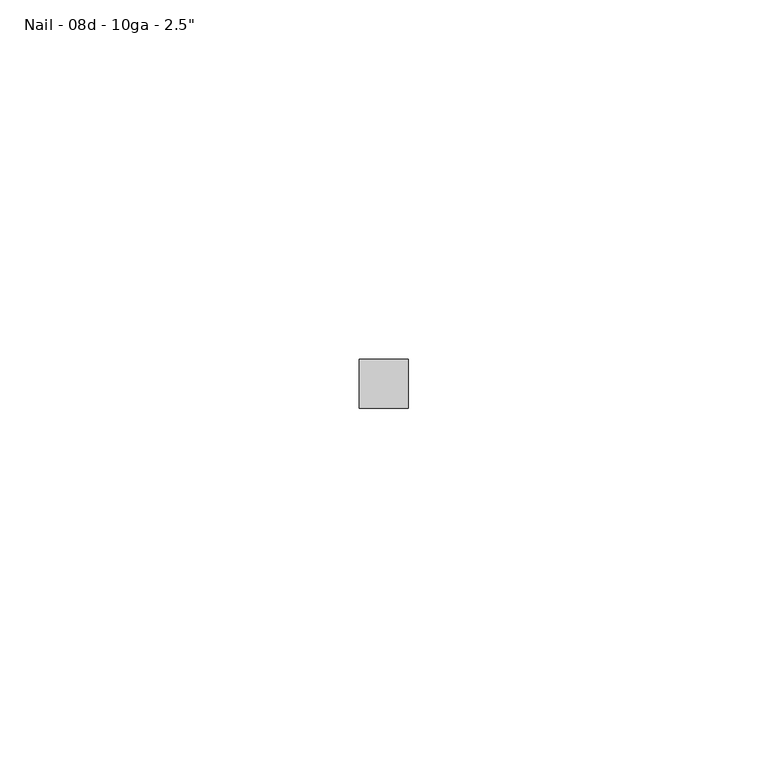
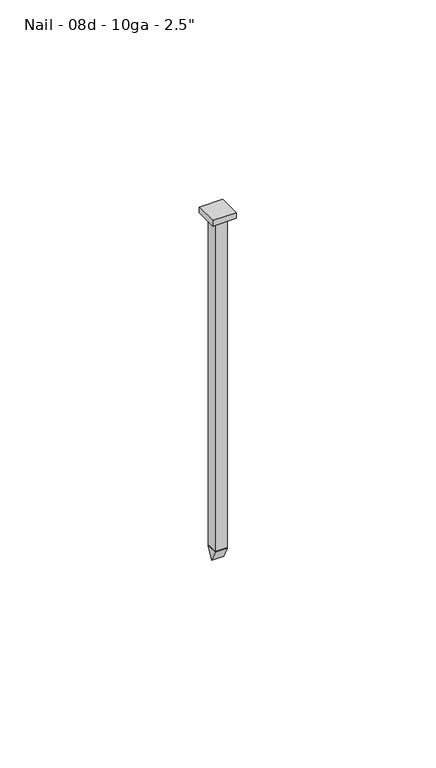
"""IFC4 building model written with IfcOpenShell, lengths in millimetres: fastener geometry."""

from ifc_helpers import new_model, si_unit, frame, origin, origin_with_axes, place, context, project, spatial, polyline, outline, extrude, source, transform, mapped, element, save


def fastener_b6cf3e51(model_context):
    return source(origin(), model_context, "Body", "SweptSolid", [
        extrude(outline(polyline([(0.0, -105.0036), (-1.7018, -101.6), (1.7018, -101.6), (0.0, -105.0036)])), frame((-1.7018, 0.0, 0.0), z_axis=(1.0, 0.0, 0.0), x_axis=(0.0, 1.0, 0.0)), (0.0, 0.0, 1.0), 3.4036),
        extrude(outline(polyline([(-3.4036, -3.4036), (-3.4036, 3.4036), (3.4036, 3.4036), (3.4036, -3.4036), (-3.4036, -3.4036)])), origin_with_axes(), (0.0, 0.0, 1.0), 1.7018),
        extrude(outline(polyline([(-1.7018, 1.7018), (1.7018, 1.7018), (1.7018, -1.7018), (-1.7018, -1.7018), (-1.7018, 1.7018)])), frame((0.0, 0.0, -101.6), z_axis=(0.0, 0.0, 1.0), x_axis=(1.0, 0.0, 0.0)), (0.0, 0.0, 1.0), 101.6),
    ])


if __name__ == "__main__":
    model = new_model("IFC4")
    model_context = context("Model", 3, world=origin())
    ifc_project = project(units=[si_unit("LENGTHUNIT", "METRE", prefix="MILLI")], contexts=[model_context])
    site = spatial("IfcSite", under=ifc_project)
    building = spatial("IfcBuilding", under=site)
    placement = place(None, origin())
    fastener_shape = fastener_b6cf3e51(model_context)
    element("IfcFastener", 1, ObjectType="060523 - W_P_C - Fastenings - Generic - SQUARE : Nail - 08d - 10ga - 2.5\"", at=placement, inside=building, context=model_context, shape_type="MappedRepresentation", body=[
        mapped(fastener_shape, transform((0.0, 0.0, 0.0), x_axis=(1.0, 0.0, 0.0), y_axis=(0.0, 1.0, 0.0), z_axis=(0.0, 0.0, 1.0))),
    ])
    save(model, "model.ifc")

# Revit data of these elements
# Type "060523 - W_P_C - Fastenings - Generic - SQUARE : Nail - 08d - 10ga - 2.5\""
#   Washer_Thickness = 0' - 0.00333"
#   Washer Radius = 0' - 0.077"
#   Washer Offset - Head = 0' - 0"
#   Washer Offset = 0' - 0"
#   Thickness_of_Substrate [instance default] = 0' - 1"
#   Side = 0' - 0 37/64"
#   Radius = 0' - 0.067"
#   Length [instance default] = 0' - 2 1/2"
#   Head Size = 0' - 1"
#   Head Radius = 0' - 0 1/2"
#   Head Height = 0' - 0.01"
#   Double Diameter = 0' - 0.268"
#   Diameter = 0' - 0.134"
#   Default Elevation = 4' - 0"
#   Washer_Nut_Visibility = no
#   Washer_Head_Visibility = no
#   Round_Head_Visibility = yes
#   Point Visibility = yes
#   Nut_Visibility = no
#   Hex_Head_Visiblilty = no
#   Washer Material = none
#   Bolt Material (Size) = AT SILL - FASTENER AT 24" O.C.
# Element 1 (IfcFastener, "060523 - W_P_C - Fastenings - Generic - SQUARE : Nail - 08d - 10ga - 2.5\"")
#   Length = 0' - 4"
# Materials
#   "AT SILL - FASTENER AT 24\" O.C.": class "Generic", colour RGB 120 120 120, transparency 0, Cost = 0
